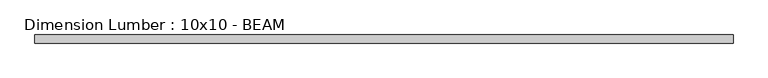
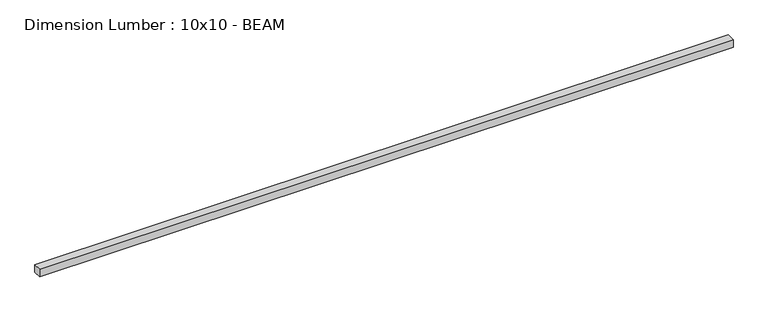
"""IFC4 building model written with IfcOpenShell, lengths in millimetres: beam geometry, Dimension Lumber : 10x10 - BEAM."""

import ifcopenshell
import ifcopenshell.guid

model = None  # the IFC model being written
_history = None  # IfcOwnerHistory: only IFC2X3 demands one
_inside = {}  # id of a spatial element -> (the spatial element, [elements in it])
_under = {}  # id of a project, library or spatial element -> (it, [spatial elements below it])
_declared = {}  # id of a project -> (the project, [libraries it declares])
_typed = {}  # id of a type object -> (the type object, [elements of that type])
_made_of = {}  # id of a material, layer set ... -> (it, [elements and type objects made of it])


def new_model(schema):
    """Start an empty IFC model of exactly this schema.

    Asked for "IFC4X3", IfcOpenShell would pick the latest addendum, in which some entities
    have other attributes; the version numbers below select the first issue.
    IFC2X3 requires an IfcOwnerHistory on every rooted entity: one is made here for all.
    """
    global model, _history
    if schema == "IFC4X3":
        model = ifcopenshell.file(schema_version=(4, 3, 0, 0))
    else:
        model = ifcopenshell.file(schema=schema)
    _inside.clear()
    _under.clear()
    _declared.clear()
    _typed.clear()
    _made_of.clear()
    _history = None
    if model.schema == "IFC2X3":
        org = make("IfcOrganization", Name="unknown")
        user = make(
            "IfcPersonAndOrganization",
            ThePerson=make("IfcPerson", FamilyName="unknown"),
            TheOrganization=org,
        )
        app = make(
            "IfcApplication",
            ApplicationDeveloper=org,
            Version="unknown",
            ApplicationFullName="unknown",
            ApplicationIdentifier="unknown",
        )
        _history = make(
            "IfcOwnerHistory",
            OwningUser=user,
            OwningApplication=app,
            ChangeAction="ADDED",
            CreationDate=0,
        )
    return model


def make(cls, **values):
    """One entity of the class cls with the attributes given. An attribute that is None is left unset."""
    return model.create_entity(
        cls, **{name: value for name, value in values.items() if value is not None}
    )


def rooted(cls, **values):
    """An entity with a GlobalId (a new one), such as an element, a storey or a relation."""
    return make(cls, GlobalId=ifcopenshell.guid.new(), OwnerHistory=_history, **values)


def si_unit(unit_type, name, prefix=None):
    """IfcSIUnit, for example si_unit("LENGTHUNIT", "METRE", prefix="MILLI")."""
    return make("IfcSIUnit", UnitType=unit_type, Prefix=prefix, Name=name)


def assignment(units):
    """IfcUnitAssignment: the units of a project."""
    return None if units is None else make("IfcUnitAssignment", Units=units)


def point(xyz):
    """IfcCartesianPoint."""
    return None if xyz is None else make("IfcCartesianPoint", Coordinates=xyz)


def direction(xyz):
    """IfcDirection."""
    return None if xyz is None else make("IfcDirection", DirectionRatios=xyz)


def frame(location, z_axis=None, x_axis=None):
    """IfcAxis2Placement3D, a coordinate frame: its origin and axes. An axis left out is left unset."""
    return make(
        "IfcAxis2Placement3D",
        Location=point(location),
        Axis=direction(z_axis),
        RefDirection=direction(x_axis),
    )


def origin():
    """The frame at (0, 0, 0) with its axes left unset."""
    return frame((0.0, 0.0, 0.0))


def place(relative_to, where):
    """IfcLocalPlacement: puts the frame where relative to a parent placement (None: the world)."""
    return make(
        "IfcLocalPlacement", PlacementRelTo=relative_to, RelativePlacement=where
    )


def context(
    kind, dimensions, precision=None, world=None, true_north=None, identifier=None
):
    """IfcGeometricRepresentationContext, for example the 3D "Model" context."""
    return make(
        "IfcGeometricRepresentationContext",
        ContextIdentifier=identifier,
        ContextType=kind,
        CoordinateSpaceDimension=dimensions,
        Precision=precision,
        WorldCoordinateSystem=world,
        TrueNorth=true_north,
    )


def project(units=None, contexts=None):
    """IfcProject with its units and contexts."""
    return rooted(
        "IfcProject",
        Name="project",
        RepresentationContexts=contexts,
        UnitsInContext=assignment(units),
    )


def spatial(cls, under=None, at=None, **own):
    """A site, building, storey or space (cls), placed at a placement, below another one or the project."""
    s = rooted(cls, ObjectPlacement=at, **own)
    if under is not None:
        _under.setdefault(under.id(), (under, []))[1].append(s)
    return s


def polyline(points):
    """IfcPolyline through the points."""
    return make("IfcPolyline", Points=[point(p) for p in points])


def outline(outer, holes=None, kind="AREA"):
    """IfcArbitraryClosedProfileDef: a profile drawn as a closed curve; with holes, ...WithVoids."""
    if holes is None:
        return make("IfcArbitraryClosedProfileDef", ProfileType=kind, OuterCurve=outer)
    return make(
        "IfcArbitraryProfileDefWithVoids",
        ProfileType=kind,
        OuterCurve=outer,
        InnerCurves=holes,
    )


def extrude(swept, where, along, depth):
    """IfcExtrudedAreaSolid: the profile swept, set in the frame where, extruded along a direction by depth."""
    return make(
        "IfcExtrudedAreaSolid",
        SweptArea=swept,
        Position=where,
        ExtrudedDirection=direction(along),
        Depth=depth,
    )


def shape(context_of_items, identifier, shape_type, items):
    """IfcShapeRepresentation: the items that make up one representation, for example the "Body"."""
    return make(
        "IfcShapeRepresentation",
        ContextOfItems=context_of_items,
        RepresentationIdentifier=identifier,
        RepresentationType=shape_type,
        Items=items,
    )


def source(mapping_origin, context_of_items, identifier, shape_type, items):
    """IfcRepresentationMap: a shape defined once, which mapped items show again and again."""
    return make(
        "IfcRepresentationMap",
        MappingOrigin=mapping_origin,
        MappedRepresentation=shape(context_of_items, identifier, shape_type, items),
    )


def transform(
    local_origin,
    x_axis=None,
    y_axis=None,
    z_axis=None,
    scale=None,
    scale2=None,
    scale3=None,
    uniform=True,
):
    """IfcCartesianTransformationOperator3D, or its non-uniform kind. x_axis, y_axis, z_axis: its Axis1, 2, 3."""
    if uniform:
        return make(
            "IfcCartesianTransformationOperator3D",
            Axis1=direction(x_axis),
            Axis2=direction(y_axis),
            LocalOrigin=point(local_origin),
            Scale=scale,
            Axis3=direction(z_axis),
        )
    return make(
        "IfcCartesianTransformationOperator3DnonUniform",
        Axis1=direction(x_axis),
        Axis2=direction(y_axis),
        LocalOrigin=point(local_origin),
        Scale=scale,
        Axis3=direction(z_axis),
        Scale2=scale2,
        Scale3=scale3,
    )


def mapped(mapping_source, mapping_target):
    """IfcMappedItem: shows the shape of a source again, moved by a transform."""
    return make(
        "IfcMappedItem", MappingSource=mapping_source, MappingTarget=mapping_target
    )


def made_of(thing, what):
    """Note that an element or type object is made of a material, layer set ...; save() writes the relation."""
    if what is not None:
        _made_of.setdefault(what.id(), (what, []))[1].append(thing)
    return thing


def element(
    cls,
    number,
    at=None,
    inside=None,
    cuts=None,
    type_object=None,
    material=None,
    context=None,
    identifier="Body",
    shape_type=None,
    held_by="IfcProductDefinitionShape",
    body=None,
    shapes=None,
    **own,
):
    """One element of the class cls, such as IfcWall. Its Tag is "e" and its number.

    at: its placement. inside: the storey or other place that contains it. cuts: it is an
    opening in that element (IfcRelVoidsElement). A single representation is given by context,
    identifier, shape_type and body (its items); several are given by shapes. held_by: the class
    of the entity that holds the representations. save() writes the other relations.
    """
    e = rooted(cls, Tag="e%d" % number, ObjectPlacement=at, **own)
    if body is not None:
        shapes = [shape(context, identifier, shape_type, body)]
    if shapes is not None:
        e.Representation = make(held_by, Representations=shapes)
    if inside is not None:
        _inside.setdefault(inside.id(), (inside, []))[1].append(e)
    if cuts is not None:
        rooted(
            "IfcRelVoidsElement", RelatingBuildingElement=cuts, RelatedOpeningElement=e
        )
    if type_object is not None:
        _typed.setdefault(type_object.id(), (type_object, []))[1].append(e)
    return made_of(e, material)


def aggregate(whole, parts):
    """IfcRelAggregates: a whole, such as a stair, and the parts it consists of."""
    return rooted("IfcRelAggregates", RelatingObject=whole, RelatedObjects=parts)


def save(model, path):
    """Write the relations noted so far, then the file.

    IfcRelAggregates (storeys below a building ...), IfcRelContainedInSpatialStructure (elements
    in a storey), IfcRelDefinesByType, IfcRelAssociatesMaterial and IfcRelDeclares: one each for
    every whole, place, type object, material and project.
    """
    for whole, parts in _under.values():
        aggregate(whole, parts)
    for where, things in _inside.values():
        rooted(
            "IfcRelContainedInSpatialStructure",
            RelatedElements=things,
            RelatingStructure=where,
        )
    for kind, things in _typed.values():
        rooted("IfcRelDefinesByType", RelatedObjects=things, RelatingType=kind)
    for what, things in _made_of.values():
        rooted("IfcRelAssociatesMaterial", RelatedObjects=things, RelatingMaterial=what)
    for by, libraries in _declared.values():
        rooted("IfcRelDeclares", RelatingContext=by, RelatedDefinitions=libraries)
    model.write(path)


def dimension_lumber_10x10_beam_1dfca716(model_context):
    return source(origin(), model_context, "Body", "SweptSolid", [
        extrude(outline(polyline([(10094.9494295, 117.475), (10094.9494295, -117.475), (-10094.9494295, -117.475), (-10094.9494295, 117.475), (10094.9494295, 117.475)])), frame((0.0, 0.0, -117.475), z_axis=(0.0, 0.0, 1.0), x_axis=(1.0, 0.0, 0.0)), (0.0, 0.0, 1.0), 234.95),
    ])


if __name__ == "__main__":
    model = new_model("IFC4")
    model_context = context("Model", 3, world=origin())
    ifc_project = project(units=[si_unit("LENGTHUNIT", "METRE", prefix="MILLI")], contexts=[model_context])
    site = spatial("IfcSite", under=ifc_project)
    building = spatial("IfcBuilding", under=site)
    placement = place(None, origin())
    dimension_lumber_10x10_beam_shape = dimension_lumber_10x10_beam_1dfca716(model_context)
    element("IfcBeam", 1, ObjectType="Dimension Lumber : 10x10 - BEAM", at=placement, inside=building, context=model_context, shape_type="MappedRepresentation", body=[
        mapped(dimension_lumber_10x10_beam_shape, transform((0.0, 0.0, 0.0), x_axis=(1.0, 0.0, 0.0), y_axis=(0.0, 1.0, 0.0), z_axis=(0.0, 0.0, 1.0))),
    ])
    save(model, "model.ifc")

# Revit data of these elements
# Type "Dimension Lumber : 10x10 - BEAM"
#   Assembly Code = "B10"
#   A = 0.0755556 SF
#   Length [instance default] = 5' - 0"
#   b = 0' - 9 1/4"
#   d = 0' - 9 1/4"
#   Structural Material = (4) CHARRED SISTERED 2X10s AT BEAM
# Element 1 (IfcBeam, "Dimension Lumber : 10x10 - BEAM")
#   Materials on its faces: "(4) CHARRED SISTERED 2X10s AT BEAM"
# Materials
#   "(4) CHARRED SISTERED 2X10s AT BEAM": class "Wood", colour RGB 144 144 144, transparency 0, Description = "Pinus Echinata", Cost = 0
